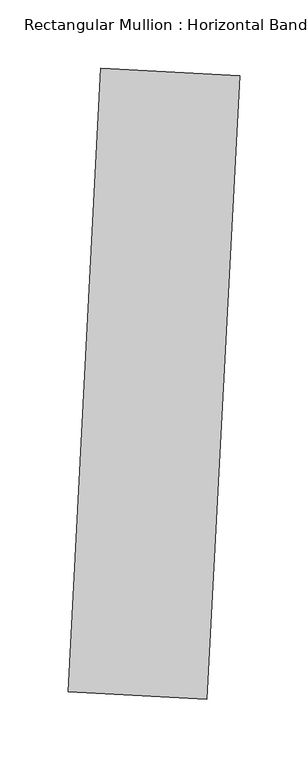
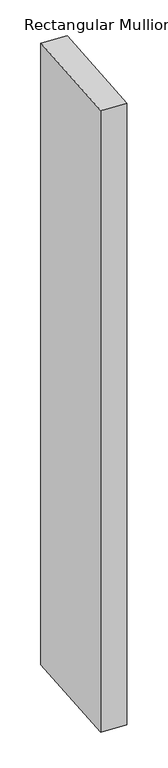
"""IFC4 building model written with IfcOpenShell, lengths in millimetres: member geometry, Rectangular Mullion : Horizontal Band."""

import ifcopenshell
import ifcopenshell.guid

model = None  # the IFC model being written
_history = None  # IfcOwnerHistory: only IFC2X3 demands one
_inside = {}  # id of a spatial element -> (the spatial element, [elements in it])
_under = {}  # id of a project, library or spatial element -> (it, [spatial elements below it])
_declared = {}  # id of a project -> (the project, [libraries it declares])
_typed = {}  # id of a type object -> (the type object, [elements of that type])
_made_of = {}  # id of a material, layer set ... -> (it, [elements and type objects made of it])


def new_model(schema):
    """Start an empty IFC model of exactly this schema.

    Asked for "IFC4X3", IfcOpenShell would pick the latest addendum, in which some entities
    have other attributes; the version numbers below select the first issue.
    IFC2X3 requires an IfcOwnerHistory on every rooted entity: one is made here for all.
    """
    global model, _history
    if schema == "IFC4X3":
        model = ifcopenshell.file(schema_version=(4, 3, 0, 0))
    else:
        model = ifcopenshell.file(schema=schema)
    _inside.clear()
    _under.clear()
    _declared.clear()
    _typed.clear()
    _made_of.clear()
    _history = None
    if model.schema == "IFC2X3":
        org = make("IfcOrganization", Name="unknown")
        user = make(
            "IfcPersonAndOrganization",
            ThePerson=make("IfcPerson", FamilyName="unknown"),
            TheOrganization=org,
        )
        app = make(
            "IfcApplication",
            ApplicationDeveloper=org,
            Version="unknown",
            ApplicationFullName="unknown",
            ApplicationIdentifier="unknown",
        )
        _history = make(
            "IfcOwnerHistory",
            OwningUser=user,
            OwningApplication=app,
            ChangeAction="ADDED",
            CreationDate=0,
        )
    return model


def make(cls, **values):
    """One entity of the class cls with the attributes given. An attribute that is None is left unset."""
    return model.create_entity(
        cls, **{name: value for name, value in values.items() if value is not None}
    )


def rooted(cls, **values):
    """An entity with a GlobalId (a new one), such as an element, a storey or a relation."""
    return make(cls, GlobalId=ifcopenshell.guid.new(), OwnerHistory=_history, **values)


def si_unit(unit_type, name, prefix=None):
    """IfcSIUnit, for example si_unit("LENGTHUNIT", "METRE", prefix="MILLI")."""
    return make("IfcSIUnit", UnitType=unit_type, Prefix=prefix, Name=name)


def assignment(units):
    """IfcUnitAssignment: the units of a project."""
    return None if units is None else make("IfcUnitAssignment", Units=units)


def point(xyz):
    """IfcCartesianPoint."""
    return None if xyz is None else make("IfcCartesianPoint", Coordinates=xyz)


def direction(xyz):
    """IfcDirection."""
    return None if xyz is None else make("IfcDirection", DirectionRatios=xyz)


def frame(location, z_axis=None, x_axis=None):
    """IfcAxis2Placement3D, a coordinate frame: its origin and axes. An axis left out is left unset."""
    return make(
        "IfcAxis2Placement3D",
        Location=point(location),
        Axis=direction(z_axis),
        RefDirection=direction(x_axis),
    )


def origin():
    """The frame at (0, 0, 0) with its axes left unset."""
    return frame((0.0, 0.0, 0.0))


def place(relative_to, where):
    """IfcLocalPlacement: puts the frame where relative to a parent placement (None: the world)."""
    return make(
        "IfcLocalPlacement", PlacementRelTo=relative_to, RelativePlacement=where
    )


def context(
    kind, dimensions, precision=None, world=None, true_north=None, identifier=None
):
    """IfcGeometricRepresentationContext, for example the 3D "Model" context."""
    return make(
        "IfcGeometricRepresentationContext",
        ContextIdentifier=identifier,
        ContextType=kind,
        CoordinateSpaceDimension=dimensions,
        Precision=precision,
        WorldCoordinateSystem=world,
        TrueNorth=true_north,
    )


def project(units=None, contexts=None):
    """IfcProject with its units and contexts."""
    return rooted(
        "IfcProject",
        Name="project",
        RepresentationContexts=contexts,
        UnitsInContext=assignment(units),
    )


def spatial(cls, under=None, at=None, **own):
    """A site, building, storey or space (cls), placed at a placement, below another one or the project."""
    s = rooted(cls, ObjectPlacement=at, **own)
    if under is not None:
        _under.setdefault(under.id(), (under, []))[1].append(s)
    return s


def polyline(points):
    """IfcPolyline through the points."""
    return make("IfcPolyline", Points=[point(p) for p in points])


def outline(outer, holes=None, kind="AREA"):
    """IfcArbitraryClosedProfileDef: a profile drawn as a closed curve; with holes, ...WithVoids."""
    if holes is None:
        return make("IfcArbitraryClosedProfileDef", ProfileType=kind, OuterCurve=outer)
    return make(
        "IfcArbitraryProfileDefWithVoids",
        ProfileType=kind,
        OuterCurve=outer,
        InnerCurves=holes,
    )


def extrude(swept, where, along, depth):
    """IfcExtrudedAreaSolid: the profile swept, set in the frame where, extruded along a direction by depth."""
    return make(
        "IfcExtrudedAreaSolid",
        SweptArea=swept,
        Position=where,
        ExtrudedDirection=direction(along),
        Depth=depth,
    )


def shape(context_of_items, identifier, shape_type, items):
    """IfcShapeRepresentation: the items that make up one representation, for example the "Body"."""
    return make(
        "IfcShapeRepresentation",
        ContextOfItems=context_of_items,
        RepresentationIdentifier=identifier,
        RepresentationType=shape_type,
        Items=items,
    )


def source(mapping_origin, context_of_items, identifier, shape_type, items):
    """IfcRepresentationMap: a shape defined once, which mapped items show again and again."""
    return make(
        "IfcRepresentationMap",
        MappingOrigin=mapping_origin,
        MappedRepresentation=shape(context_of_items, identifier, shape_type, items),
    )


def transform(
    local_origin,
    x_axis=None,
    y_axis=None,
    z_axis=None,
    scale=None,
    scale2=None,
    scale3=None,
    uniform=True,
):
    """IfcCartesianTransformationOperator3D, or its non-uniform kind. x_axis, y_axis, z_axis: its Axis1, 2, 3."""
    if uniform:
        return make(
            "IfcCartesianTransformationOperator3D",
            Axis1=direction(x_axis),
            Axis2=direction(y_axis),
            LocalOrigin=point(local_origin),
            Scale=scale,
            Axis3=direction(z_axis),
        )
    return make(
        "IfcCartesianTransformationOperator3DnonUniform",
        Axis1=direction(x_axis),
        Axis2=direction(y_axis),
        LocalOrigin=point(local_origin),
        Scale=scale,
        Axis3=direction(z_axis),
        Scale2=scale2,
        Scale3=scale3,
    )


def mapped(mapping_source, mapping_target):
    """IfcMappedItem: shows the shape of a source again, moved by a transform."""
    return make(
        "IfcMappedItem", MappingSource=mapping_source, MappingTarget=mapping_target
    )


def made_of(thing, what):
    """Note that an element or type object is made of a material, layer set ...; save() writes the relation."""
    if what is not None:
        _made_of.setdefault(what.id(), (what, []))[1].append(thing)
    return thing


def element(
    cls,
    number,
    at=None,
    inside=None,
    cuts=None,
    type_object=None,
    material=None,
    context=None,
    identifier="Body",
    shape_type=None,
    held_by="IfcProductDefinitionShape",
    body=None,
    shapes=None,
    **own,
):
    """One element of the class cls, such as IfcWall. Its Tag is "e" and its number.

    at: its placement. inside: the storey or other place that contains it. cuts: it is an
    opening in that element (IfcRelVoidsElement). A single representation is given by context,
    identifier, shape_type and body (its items); several are given by shapes. held_by: the class
    of the entity that holds the representations. save() writes the other relations.
    """
    e = rooted(cls, Tag="e%d" % number, ObjectPlacement=at, **own)
    if body is not None:
        shapes = [shape(context, identifier, shape_type, body)]
    if shapes is not None:
        e.Representation = make(held_by, Representations=shapes)
    if inside is not None:
        _inside.setdefault(inside.id(), (inside, []))[1].append(e)
    if cuts is not None:
        rooted(
            "IfcRelVoidsElement", RelatingBuildingElement=cuts, RelatedOpeningElement=e
        )
    if type_object is not None:
        _typed.setdefault(type_object.id(), (type_object, []))[1].append(e)
    return made_of(e, material)


def aggregate(whole, parts):
    """IfcRelAggregates: a whole, such as a stair, and the parts it consists of."""
    return rooted("IfcRelAggregates", RelatingObject=whole, RelatedObjects=parts)


def save(model, path):
    """Write the relations noted so far, then the file.

    IfcRelAggregates (storeys below a building ...), IfcRelContainedInSpatialStructure (elements
    in a storey), IfcRelDefinesByType, IfcRelAssociatesMaterial and IfcRelDeclares: one each for
    every whole, place, type object, material and project.
    """
    for whole, parts in _under.values():
        aggregate(whole, parts)
    for where, things in _inside.values():
        rooted(
            "IfcRelContainedInSpatialStructure",
            RelatedElements=things,
            RelatingStructure=where,
        )
    for kind, things in _typed.values():
        rooted("IfcRelDefinesByType", RelatedObjects=things, RelatingType=kind)
    for what, things in _made_of.values():
        rooted("IfcRelAssociatesMaterial", RelatedObjects=things, RelatingMaterial=what)
    for by, libraries in _declared.values():
        rooted("IfcRelDeclares", RelatingContext=by, RelatedDefinitions=libraries)
    model.write(path)


def rectangular_mullion_horizontal_band_87718f43(model_context):
    return source(origin(), model_context, "Body", "SweptSolid", [
        extrude(outline(polyline([(62.69438, 301.8280451), (38.7663808, -154.7453782), (-62.69438, -149.4280451), (-38.7663808, 307.1453782), (62.69438, 301.8280451)])), frame((0.0, 0.0, -2629.1291719), z_axis=(0.0, 0.0, 1.0), x_axis=(1.0, 0.0, 0.0)), (0.0, 0.0, 1.0), 2629.1291719),
    ])


if __name__ == "__main__":
    model = new_model("IFC4")
    model_context = context("Model", 3, world=origin())
    ifc_project = project(units=[si_unit("LENGTHUNIT", "METRE", prefix="MILLI")], contexts=[model_context])
    site = spatial("IfcSite", under=ifc_project)
    building = spatial("IfcBuilding", under=site)
    placement = place(None, origin())
    rectangular_mullion_horizontal_band_shape = rectangular_mullion_horizontal_band_87718f43(model_context)
    element("IfcMember", 1, ObjectType="Rectangular Mullion : Horizontal Band", at=placement, inside=building, context=model_context, shape_type="MappedRepresentation", body=[
        mapped(rectangular_mullion_horizontal_band_shape, transform((0.0, 0.0, 0.0), x_axis=(1.0, 0.0, 0.0), y_axis=(0.0, 1.0, 0.0), z_axis=(0.0, 0.0, 1.0))),
    ])
    save(model, "model.ifc")

# Revit data of these elements
# Type "Rectangular Mullion : Horizontal Band"
#   built-in parameter 1007351 = 0.25 (stored number, unit not read)
#   built-in parameter 1007304 = 1.5 (stored number, unit not read)
#   built-in parameter 1007301 = 0.166667 (stored number, unit not read)
#   built-in parameter 1007300 = 0.166667 (stored number, unit not read)
# Element 1 (IfcMember, "Rectangular Mullion : Horizontal Band")
#   Materials on its faces: "Aluminum"
# Materials
#   "Aluminum": class "Metal", colour RGB 247 247 247, transparency 0, Description = "Aluminum 6061", Cost = 0
